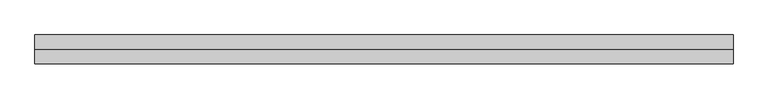
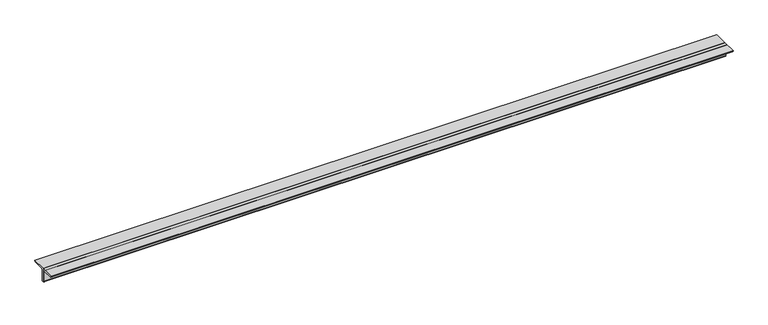
"""IFC4 building model written with IfcOpenShell, lengths in millimetres: member geometry, 0123_Steel Framing_2Ls-KSD3502 : H_SB_AR_S04_2Ls-130x130x12_VBR2."""

from ifc_helpers import new_model, si_unit, point, frame, frame_2d, origin, place, context, project, spatial, polyline, circle_curve, trimmed, segment, composite_curve, outline, extrude, source, transform, mapped, element, save


def member_08074ba6(model_context):
    return source(origin(), model_context, "Body", "SweptSolid", [
        extrude(outline(composite_curve([segment(polyline([(0.0, 36.4), (130.0, 36.4)]), True, "CONTINUOUS"), segment(trimmed(circle_curve(frame_2d((118.0, 36.4)), 12.0), [point((130.0, 36.4))], [point((118.0, 24.4))], False, "CARTESIAN"), True, "CONTINUOUS"), segment(polyline([(118.0, 24.4), (24.0, 24.4)]), True, "CONTINUOUS"), segment(trimmed(circle_curve(frame_2d((24.0, 12.4)), 12.0), [point((24.0, 24.4))], [point((12.0, 12.4))], True, "CARTESIAN"), True, "CONTINUOUS"), segment(polyline([(12.0, 12.4), (12.0, -81.6)]), True, "CONTINUOUS"), segment(trimmed(circle_curve(frame_2d((0.0, -81.6)), 12.0), [point((12.0, -81.6))], [point((0.0, -93.6))], False, "CARTESIAN"), True, "CONTINUOUS"), segment(polyline([(0.0, -93.6), (0.0, 36.4)]), True, "CONTINUOUS")], self_intersect=False)), frame((-2961.9806044, 0.0, 0.0), z_axis=(1.0, 0.0, 0.0), x_axis=(0.0, 1.0, 0.0)), (0.0, 0.0, 1.0), 6322.5847795),
        extrude(outline(composite_curve([segment(polyline([(0.0, 36.4), (0.0, -93.6)]), True, "CONTINUOUS"), segment(trimmed(circle_curve(frame_2d((0.0, -81.6)), 12.0), [point((0.0, -93.6))], [point((-12.0, -81.6))], False, "CARTESIAN"), True, "CONTINUOUS"), segment(polyline([(-12.0, -81.6), (-12.0, 12.4)]), True, "CONTINUOUS"), segment(trimmed(circle_curve(frame_2d((-24.0, 12.4)), 12.0), [point((-12.0, 12.4))], [point((-24.0, 24.4))], True, "CARTESIAN"), True, "CONTINUOUS"), segment(polyline([(-24.0, 24.4), (-118.0, 24.4)]), True, "CONTINUOUS"), segment(trimmed(circle_curve(frame_2d((-118.0, 36.4)), 12.0), [point((-118.0, 24.4))], [point((-130.0, 36.4))], False, "CARTESIAN"), True, "CONTINUOUS"), segment(polyline([(-130.0, 36.4), (0.0, 36.4)]), True, "CONTINUOUS")], self_intersect=False)), frame((-2961.9806044, 0.0, 0.0), z_axis=(1.0, 0.0, 0.0), x_axis=(0.0, 1.0, 0.0)), (0.0, 0.0, 1.0), 6322.5847795),
    ])


if __name__ == "__main__":
    model = new_model("IFC4")
    model_context = context("Model", 3, world=origin())
    ifc_project = project(units=[si_unit("LENGTHUNIT", "METRE", prefix="MILLI")], contexts=[model_context])
    site = spatial("IfcSite", under=ifc_project)
    building = spatial("IfcBuilding", under=site)
    placement = place(None, origin())
    member_shape = member_08074ba6(model_context)
    element("IfcMember", 1, ObjectType="0123_Steel Framing_2Ls-KSD3502 : H_SB_AR_S04_2Ls-130x130x12_VBR2", at=placement, inside=building, context=model_context, shape_type="MappedRepresentation", body=[
        mapped(member_shape, transform((0.0, 0.0, 0.0), x_axis=(1.0, 0.0, 0.0), y_axis=(0.0, 1.0, 0.0), z_axis=(0.0, 0.0, 1.0))),
    ])
    save(model, "model.ifc")

# Revit data of these elements
# Type "0123_Steel Framing_2Ls-KSD3502 : H_SB_AR_S04_2Ls-130x130x12_VBR2"
#   Assembly Code = "B10"
#   Legs = "SLBB"
#   W = 8.97
#   Perimeter = 1.04 m²/m
#   Nominal Weight = 46.80 kgf/m
#   Length [instance default] = 1000 mm
#   Space = 0 mm
#   b = 130 mm
#   d = 130 mm
#   t = 12 mm
#   y = 36.4 mm
#   A = 0.005952 m²
#   Structural Material [instance default] = Steel ASTM A36
# Element 1 (IfcMember, "0123_Steel Framing_2Ls-KSD3502 : H_SB_AR_S04_2Ls-130x130x12_VBR2")
#   Structural Material = Steel, 45-345
#   Materials on its faces: "Steel, 45-345"
# Materials
#   "Steel ASTM A36": class "Metal", colour RGB 199 199 199, transparency 0, Description = "Structural steel, ASTM A36 Grade B, mill finish", Cost = 0
#   "Steel, 45-345": class "Metal", colour RGB 189 187 185, transparency 0, Description = "Steel 345 MPa", Cost = 0
